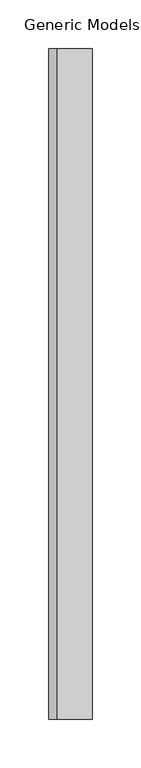
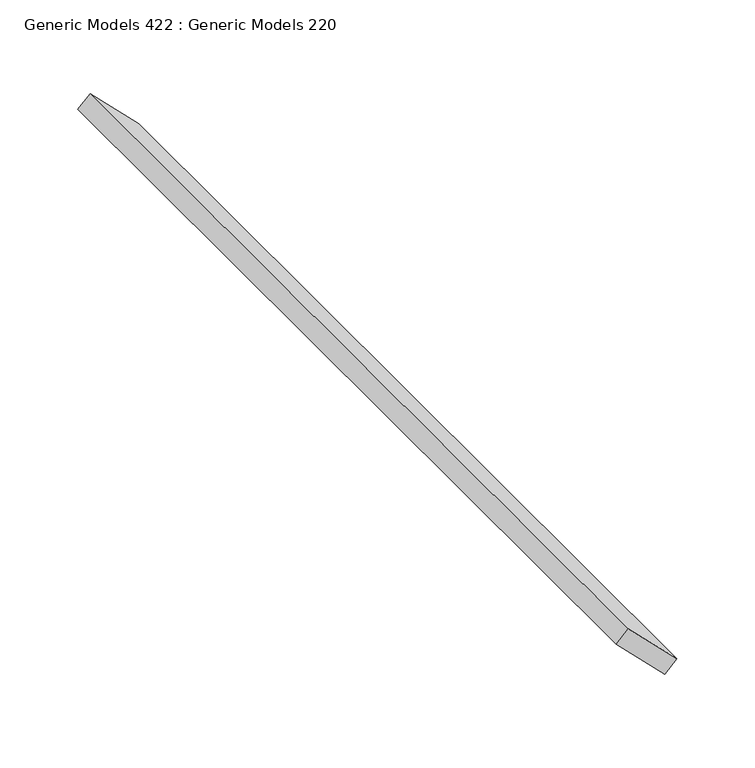
"""IFC4 building model written with IfcOpenShell, lengths in millimetres: proxy geometry, Generic Models 422 : Generic Models 220."""

from ifc_helpers import new_model, si_unit, frame, origin, place, context, project, spatial, polyline, outline, extrude, source, transform, mapped, element, save


def generic_models_422_generic_models_220_3abe8308(model_context):
    return source(origin(), model_context, "Body", "SweptSolid", [
        extrude(outline(polyline([(0.0, -50.8), (0.0, 0.0), (690.8142348, 0.0), (690.8142348, -50.8), (0.0, -50.8)])), frame((-6899.085451, -4564.8872686, 128577.1762561), z_axis=(0.7071067811865582, 0.0, 0.7071067811865369), x_axis=(0.0, 1.0, 0.0)), (0.0, 0.0, 1.0), 12.7),
    ])


if __name__ == "__main__":
    model = new_model("IFC4")
    model_context = context("Model", 3, world=origin())
    ifc_project = project(units=[si_unit("LENGTHUNIT", "METRE", prefix="MILLI")], contexts=[model_context])
    site = spatial("IfcSite", under=ifc_project)
    building = spatial("IfcBuilding", under=site)
    placement = place(None, origin())
    generic_models_422_generic_models_220_shape = generic_models_422_generic_models_220_3abe8308(model_context)
    element("IfcBuildingElementProxy", 1, Name="Generic Models 422 : Generic Models 220", ObjectType="Generic Models 422 : Generic Models 220", at=placement, inside=building, context=model_context, shape_type="MappedRepresentation", body=[
        mapped(generic_models_422_generic_models_220_shape, transform((0.0, 0.0, 0.0), x_axis=(1.0, 0.0, 0.0), y_axis=(0.0, 1.0, 0.0), z_axis=(0.0, 0.0, 1.0))),
    ])
    save(model, "model.ifc")

# Revit data of these elements
# Element 1 (IfcBuildingElementProxy, "Generic Models 422 : Generic Models 220")
#   Materials on its faces: "_WOOD TONE ALUMINUM EXTRUSION SLAT BY KNOTWOOD"
# Materials
#   "_WOOD TONE ALUMINUM EXTRUSION SLAT BY KNOTWOOD": class "Generic", colour RGB 177 130 114, transparency 0, Cost = 0
